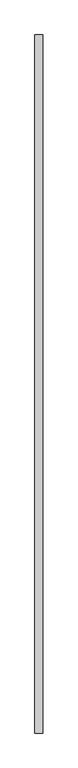
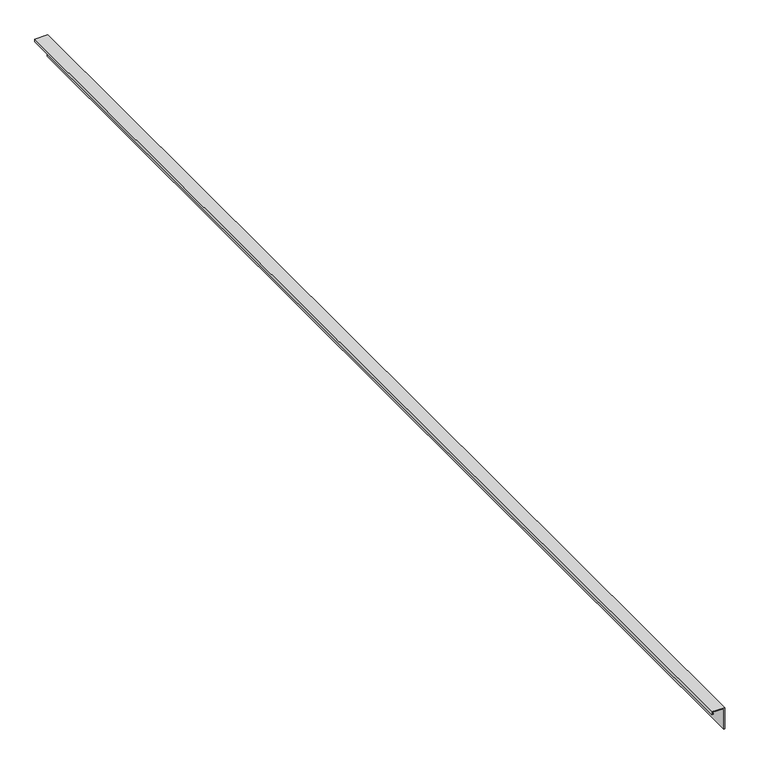
"""IFC4 building model written with IfcOpenShell, lengths in millimetres: proxy geometry, GRAVEL STOP12:GRAVEL STOP003:299952 : GRAVEL STOP12:GRAVEL STOP003:299952."""

import ifcopenshell
import ifcopenshell.guid

model = None  # the IFC model being written
_history = None  # IfcOwnerHistory: only IFC2X3 demands one
_inside = {}  # id of a spatial element -> (the spatial element, [elements in it])
_under = {}  # id of a project, library or spatial element -> (it, [spatial elements below it])
_declared = {}  # id of a project -> (the project, [libraries it declares])
_typed = {}  # id of a type object -> (the type object, [elements of that type])
_made_of = {}  # id of a material, layer set ... -> (it, [elements and type objects made of it])


def new_model(schema):
    """Start an empty IFC model of exactly this schema.

    Asked for "IFC4X3", IfcOpenShell would pick the latest addendum, in which some entities
    have other attributes; the version numbers below select the first issue.
    IFC2X3 requires an IfcOwnerHistory on every rooted entity: one is made here for all.
    """
    global model, _history
    if schema == "IFC4X3":
        model = ifcopenshell.file(schema_version=(4, 3, 0, 0))
    else:
        model = ifcopenshell.file(schema=schema)
    _inside.clear()
    _under.clear()
    _declared.clear()
    _typed.clear()
    _made_of.clear()
    _history = None
    if model.schema == "IFC2X3":
        org = make("IfcOrganization", Name="unknown")
        user = make(
            "IfcPersonAndOrganization",
            ThePerson=make("IfcPerson", FamilyName="unknown"),
            TheOrganization=org,
        )
        app = make(
            "IfcApplication",
            ApplicationDeveloper=org,
            Version="unknown",
            ApplicationFullName="unknown",
            ApplicationIdentifier="unknown",
        )
        _history = make(
            "IfcOwnerHistory",
            OwningUser=user,
            OwningApplication=app,
            ChangeAction="ADDED",
            CreationDate=0,
        )
    return model


def make(cls, **values):
    """One entity of the class cls with the attributes given. An attribute that is None is left unset."""
    return model.create_entity(
        cls, **{name: value for name, value in values.items() if value is not None}
    )


def rooted(cls, **values):
    """An entity with a GlobalId (a new one), such as an element, a storey or a relation."""
    return make(cls, GlobalId=ifcopenshell.guid.new(), OwnerHistory=_history, **values)


def si_unit(unit_type, name, prefix=None):
    """IfcSIUnit, for example si_unit("LENGTHUNIT", "METRE", prefix="MILLI")."""
    return make("IfcSIUnit", UnitType=unit_type, Prefix=prefix, Name=name)


def assignment(units):
    """IfcUnitAssignment: the units of a project."""
    return None if units is None else make("IfcUnitAssignment", Units=units)


def point(xyz):
    """IfcCartesianPoint."""
    return None if xyz is None else make("IfcCartesianPoint", Coordinates=xyz)


def direction(xyz):
    """IfcDirection."""
    return None if xyz is None else make("IfcDirection", DirectionRatios=xyz)


def frame(location, z_axis=None, x_axis=None):
    """IfcAxis2Placement3D, a coordinate frame: its origin and axes. An axis left out is left unset."""
    return make(
        "IfcAxis2Placement3D",
        Location=point(location),
        Axis=direction(z_axis),
        RefDirection=direction(x_axis),
    )


def origin():
    """The frame at (0, 0, 0) with its axes left unset."""
    return frame((0.0, 0.0, 0.0))


def place(relative_to, where):
    """IfcLocalPlacement: puts the frame where relative to a parent placement (None: the world)."""
    return make(
        "IfcLocalPlacement", PlacementRelTo=relative_to, RelativePlacement=where
    )


def context(
    kind, dimensions, precision=None, world=None, true_north=None, identifier=None
):
    """IfcGeometricRepresentationContext, for example the 3D "Model" context."""
    return make(
        "IfcGeometricRepresentationContext",
        ContextIdentifier=identifier,
        ContextType=kind,
        CoordinateSpaceDimension=dimensions,
        Precision=precision,
        WorldCoordinateSystem=world,
        TrueNorth=true_north,
    )


def project(units=None, contexts=None):
    """IfcProject with its units and contexts."""
    return rooted(
        "IfcProject",
        Name="project",
        RepresentationContexts=contexts,
        UnitsInContext=assignment(units),
    )


def spatial(cls, under=None, at=None, **own):
    """A site, building, storey or space (cls), placed at a placement, below another one or the project."""
    s = rooted(cls, ObjectPlacement=at, **own)
    if under is not None:
        _under.setdefault(under.id(), (under, []))[1].append(s)
    return s


def polyline(points):
    """IfcPolyline through the points."""
    return make("IfcPolyline", Points=[point(p) for p in points])


def outline(outer, holes=None, kind="AREA"):
    """IfcArbitraryClosedProfileDef: a profile drawn as a closed curve; with holes, ...WithVoids."""
    if holes is None:
        return make("IfcArbitraryClosedProfileDef", ProfileType=kind, OuterCurve=outer)
    return make(
        "IfcArbitraryProfileDefWithVoids",
        ProfileType=kind,
        OuterCurve=outer,
        InnerCurves=holes,
    )


def extrude(swept, where, along, depth):
    """IfcExtrudedAreaSolid: the profile swept, set in the frame where, extruded along a direction by depth."""
    return make(
        "IfcExtrudedAreaSolid",
        SweptArea=swept,
        Position=where,
        ExtrudedDirection=direction(along),
        Depth=depth,
    )


def shape(context_of_items, identifier, shape_type, items):
    """IfcShapeRepresentation: the items that make up one representation, for example the "Body"."""
    return make(
        "IfcShapeRepresentation",
        ContextOfItems=context_of_items,
        RepresentationIdentifier=identifier,
        RepresentationType=shape_type,
        Items=items,
    )


def source(mapping_origin, context_of_items, identifier, shape_type, items):
    """IfcRepresentationMap: a shape defined once, which mapped items show again and again."""
    return make(
        "IfcRepresentationMap",
        MappingOrigin=mapping_origin,
        MappedRepresentation=shape(context_of_items, identifier, shape_type, items),
    )


def transform(
    local_origin,
    x_axis=None,
    y_axis=None,
    z_axis=None,
    scale=None,
    scale2=None,
    scale3=None,
    uniform=True,
):
    """IfcCartesianTransformationOperator3D, or its non-uniform kind. x_axis, y_axis, z_axis: its Axis1, 2, 3."""
    if uniform:
        return make(
            "IfcCartesianTransformationOperator3D",
            Axis1=direction(x_axis),
            Axis2=direction(y_axis),
            LocalOrigin=point(local_origin),
            Scale=scale,
            Axis3=direction(z_axis),
        )
    return make(
        "IfcCartesianTransformationOperator3DnonUniform",
        Axis1=direction(x_axis),
        Axis2=direction(y_axis),
        LocalOrigin=point(local_origin),
        Scale=scale,
        Axis3=direction(z_axis),
        Scale2=scale2,
        Scale3=scale3,
    )


def mapped(mapping_source, mapping_target):
    """IfcMappedItem: shows the shape of a source again, moved by a transform."""
    return make(
        "IfcMappedItem", MappingSource=mapping_source, MappingTarget=mapping_target
    )


def made_of(thing, what):
    """Note that an element or type object is made of a material, layer set ...; save() writes the relation."""
    if what is not None:
        _made_of.setdefault(what.id(), (what, []))[1].append(thing)
    return thing


def element(
    cls,
    number,
    at=None,
    inside=None,
    cuts=None,
    type_object=None,
    material=None,
    context=None,
    identifier="Body",
    shape_type=None,
    held_by="IfcProductDefinitionShape",
    body=None,
    shapes=None,
    **own,
):
    """One element of the class cls, such as IfcWall. Its Tag is "e" and its number.

    at: its placement. inside: the storey or other place that contains it. cuts: it is an
    opening in that element (IfcRelVoidsElement). A single representation is given by context,
    identifier, shape_type and body (its items); several are given by shapes. held_by: the class
    of the entity that holds the representations. save() writes the other relations.
    """
    e = rooted(cls, Tag="e%d" % number, ObjectPlacement=at, **own)
    if body is not None:
        shapes = [shape(context, identifier, shape_type, body)]
    if shapes is not None:
        e.Representation = make(held_by, Representations=shapes)
    if inside is not None:
        _inside.setdefault(inside.id(), (inside, []))[1].append(e)
    if cuts is not None:
        rooted(
            "IfcRelVoidsElement", RelatingBuildingElement=cuts, RelatedOpeningElement=e
        )
    if type_object is not None:
        _typed.setdefault(type_object.id(), (type_object, []))[1].append(e)
    return made_of(e, material)


def aggregate(whole, parts):
    """IfcRelAggregates: a whole, such as a stair, and the parts it consists of."""
    return rooted("IfcRelAggregates", RelatingObject=whole, RelatedObjects=parts)


def save(model, path):
    """Write the relations noted so far, then the file.

    IfcRelAggregates (storeys below a building ...), IfcRelContainedInSpatialStructure (elements
    in a storey), IfcRelDefinesByType, IfcRelAssociatesMaterial and IfcRelDeclares: one each for
    every whole, place, type object, material and project.
    """
    for whole, parts in _under.values():
        aggregate(whole, parts)
    for where, things in _inside.values():
        rooted(
            "IfcRelContainedInSpatialStructure",
            RelatedElements=things,
            RelatingStructure=where,
        )
    for kind, things in _typed.values():
        rooted("IfcRelDefinesByType", RelatedObjects=things, RelatingType=kind)
    for what, things in _made_of.values():
        rooted("IfcRelAssociatesMaterial", RelatedObjects=things, RelatingMaterial=what)
    for by, libraries in _declared.values():
        rooted("IfcRelDeclares", RelatingContext=by, RelatedDefinitions=libraries)
    model.write(path)


def generic_models_73a3dd64(model_context):
    return source(origin(), model_context, "Body", "SweptSolid", [
        extrude(outline(polyline([(40234.4061757, -263.93472), (40234.4061757, -244.24972), (40197.5761757, -244.24972), (40197.5761757, -242.97972), (40235.6761757, -242.97972), (40235.6761757, -265.20472), (40230.9263757, -265.20472), (40230.9263757, -262.2022636), (40232.1963757, -262.2022636), (40232.1963757, -263.93472), (40234.4061757, -263.93472)])), frame((0.0, -774.5581162, 0.0), z_axis=(0.0, 1.0, 0.0), x_axis=(0.0, 0.0, 1.0)), (0.0, 0.0, 1.0), 2000.25),
    ])


if __name__ == "__main__":
    model = new_model("IFC4")
    model_context = context("Model", 3, world=origin())
    ifc_project = project(units=[si_unit("LENGTHUNIT", "METRE", prefix="MILLI")], contexts=[model_context])
    site = spatial("IfcSite", under=ifc_project)
    building = spatial("IfcBuilding", under=site)
    placement = place(None, origin())
    generic_models_shape = generic_models_73a3dd64(model_context)
    element("IfcBuildingElementProxy", 1, Name="GRAVEL STOP12:GRAVEL STOP003:299952 : GRAVEL STOP12:GRAVEL STOP003:299952", ObjectType="GRAVEL STOP12:GRAVEL STOP003:299952 : GRAVEL STOP12:GRAVEL STOP003:299952", at=placement, inside=building, context=model_context, shape_type="MappedRepresentation", body=[
        mapped(generic_models_shape, transform((0.0, 0.0, 0.0), x_axis=(1.0, 0.0, 0.0), y_axis=(0.0, 1.0, 0.0), z_axis=(0.0, 0.0, 1.0))),
    ])
    save(model, "model.ifc")

# Revit data of these elements
# Type "GRAVEL STOP12:GRAVEL STOP003:299952 : GRAVEL STOP12:GRAVEL STOP003:299952"
#   NameOverride = "GRAVEL STOP12:GRAVEL STOP003:299952"
#   ObjectTypeOverride = "GRAVEL STOP12:GRAVEL STOP003"
#   Reference = "GRAVEL STOP003"
#   Category = "Generic Models"
#   Tag = "299952"
# Element 1 (IfcBuildingElementProxy, "GRAVEL STOP12:GRAVEL STOP003:299952 : GRAVEL STOP12:GRAVEL STOP003:299952")
#   Materials on its faces: "COPPER STUCCO J BEAD"
# Materials
#   "COPPER STUCCO J BEAD": class "Unassigned", colour RGB 251 232 155, transparency 0, Cost = 0
